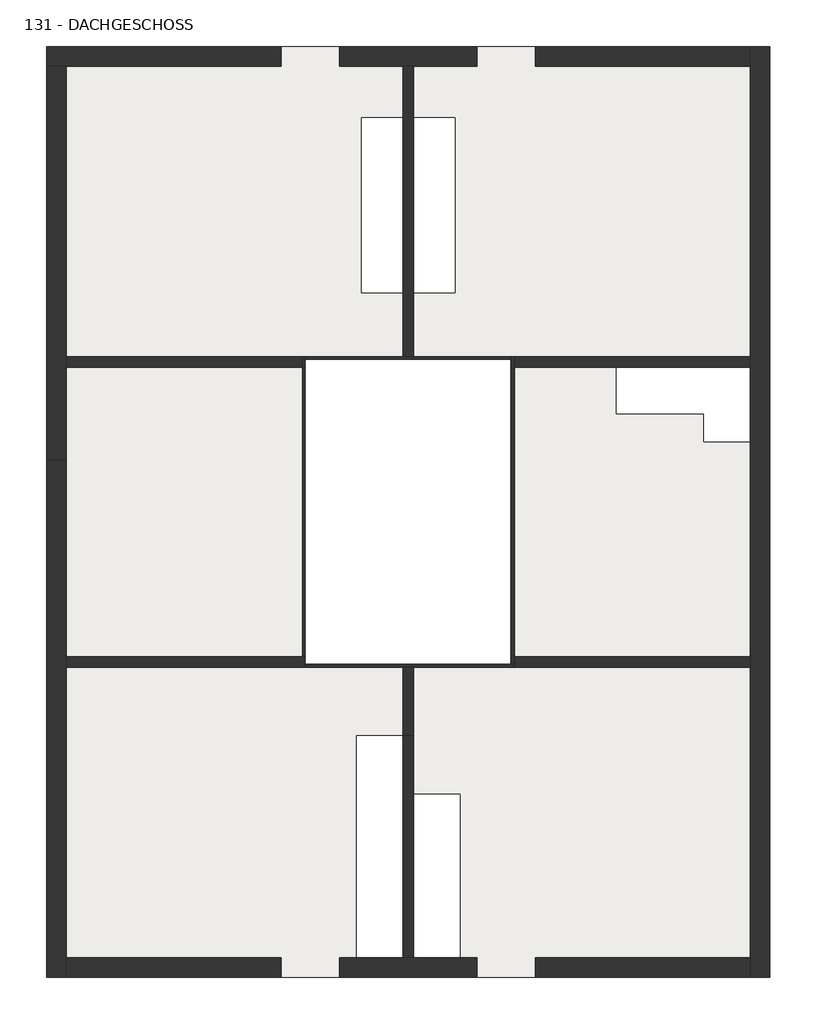
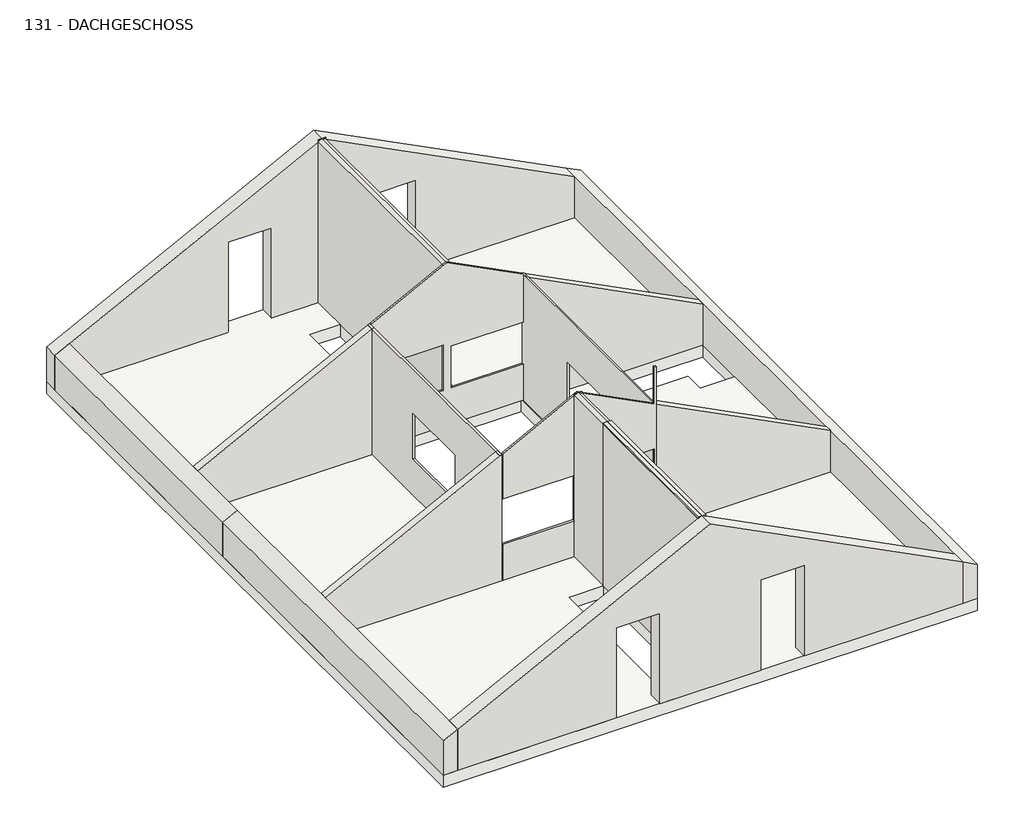
# One storey: 16 walls, 1 slab.
"""IFC4 building model written with IfcOpenShell, lengths in millimetres."""

import ifcopenshell
import ifcopenshell.guid

model = None  # the IFC model being written
_history = None  # IfcOwnerHistory: only IFC2X3 demands one
_inside = {}  # id of a spatial element -> (the spatial element, [elements in it])
_under = {}  # id of a project, library or spatial element -> (it, [spatial elements below it])
_declared = {}  # id of a project -> (the project, [libraries it declares])
_typed = {}  # id of a type object -> (the type object, [elements of that type])
_made_of = {}  # id of a material, layer set ... -> (it, [elements and type objects made of it])


def new_model(schema):
    """Start an empty IFC model of exactly this schema.

    Asked for "IFC4X3", IfcOpenShell would pick the latest addendum, in which some entities
    have other attributes; the version numbers below select the first issue.
    IFC2X3 requires an IfcOwnerHistory on every rooted entity: one is made here for all.
    """
    global model, _history
    if schema == "IFC4X3":
        model = ifcopenshell.file(schema_version=(4, 3, 0, 0))
    else:
        model = ifcopenshell.file(schema=schema)
    _inside.clear()
    _under.clear()
    _declared.clear()
    _typed.clear()
    _made_of.clear()
    _history = None
    if model.schema == "IFC2X3":
        org = make("IfcOrganization", Name="unknown")
        user = make(
            "IfcPersonAndOrganization",
            ThePerson=make("IfcPerson", FamilyName="unknown"),
            TheOrganization=org,
        )
        app = make(
            "IfcApplication",
            ApplicationDeveloper=org,
            Version="unknown",
            ApplicationFullName="unknown",
            ApplicationIdentifier="unknown",
        )
        _history = make(
            "IfcOwnerHistory",
            OwningUser=user,
            OwningApplication=app,
            ChangeAction="ADDED",
            CreationDate=0,
        )
    return model


def make(cls, **values):
    """One entity of the class cls with the attributes given. An attribute that is None is left unset."""
    return model.create_entity(
        cls, **{name: value for name, value in values.items() if value is not None}
    )


def rooted(cls, **values):
    """An entity with a GlobalId (a new one), such as an element, a storey or a relation."""
    return make(cls, GlobalId=ifcopenshell.guid.new(), OwnerHistory=_history, **values)


def si_unit(unit_type, name, prefix=None):
    """IfcSIUnit, for example si_unit("LENGTHUNIT", "METRE", prefix="MILLI")."""
    return make("IfcSIUnit", UnitType=unit_type, Prefix=prefix, Name=name)


def assignment(units):
    """IfcUnitAssignment: the units of a project."""
    return None if units is None else make("IfcUnitAssignment", Units=units)


def point(xyz):
    """IfcCartesianPoint."""
    return None if xyz is None else make("IfcCartesianPoint", Coordinates=xyz)


def direction(xyz):
    """IfcDirection."""
    return None if xyz is None else make("IfcDirection", DirectionRatios=xyz)


def frame(location, z_axis=None, x_axis=None):
    """IfcAxis2Placement3D, a coordinate frame: its origin and axes. An axis left out is left unset."""
    return make(
        "IfcAxis2Placement3D",
        Location=point(location),
        Axis=direction(z_axis),
        RefDirection=direction(x_axis),
    )


def origin():
    """The frame at (0, 0, 0) with its axes left unset."""
    return frame((0.0, 0.0, 0.0))


def place(relative_to, where):
    """IfcLocalPlacement: puts the frame where relative to a parent placement (None: the world)."""
    return make(
        "IfcLocalPlacement", PlacementRelTo=relative_to, RelativePlacement=where
    )


def context(
    kind, dimensions, precision=None, world=None, true_north=None, identifier=None
):
    """IfcGeometricRepresentationContext, for example the 3D "Model" context."""
    return make(
        "IfcGeometricRepresentationContext",
        ContextIdentifier=identifier,
        ContextType=kind,
        CoordinateSpaceDimension=dimensions,
        Precision=precision,
        WorldCoordinateSystem=world,
        TrueNorth=true_north,
    )


def project(units=None, contexts=None):
    """IfcProject with its units and contexts."""
    return rooted(
        "IfcProject",
        Name="project",
        RepresentationContexts=contexts,
        UnitsInContext=assignment(units),
    )


def spatial(cls, under=None, at=None, **own):
    """A site, building, storey or space (cls), placed at a placement, below another one or the project."""
    s = rooted(cls, ObjectPlacement=at, **own)
    if under is not None:
        _under.setdefault(under.id(), (under, []))[1].append(s)
    return s


def polyline(points):
    """IfcPolyline through the points."""
    return make("IfcPolyline", Points=[point(p) for p in points])


def outline(outer, holes=None, kind="AREA"):
    """IfcArbitraryClosedProfileDef: a profile drawn as a closed curve; with holes, ...WithVoids."""
    if holes is None:
        return make("IfcArbitraryClosedProfileDef", ProfileType=kind, OuterCurve=outer)
    return make(
        "IfcArbitraryProfileDefWithVoids",
        ProfileType=kind,
        OuterCurve=outer,
        InnerCurves=holes,
    )


def extrude(swept, where, along, depth):
    """IfcExtrudedAreaSolid: the profile swept, set in the frame where, extruded along a direction by depth."""
    return make(
        "IfcExtrudedAreaSolid",
        SweptArea=swept,
        Position=where,
        ExtrudedDirection=direction(along),
        Depth=depth,
    )


def faces_of(points, faces, orient=None, outer=None):
    """IfcFace entities. A face is a list of loops; a loop is a list of indices into points, from 0.

    orient and outer hold one flag for each loop. By default every Orientation is true, the
    first loop of a face is its IfcFaceOuterBound and the others are IfcFaceBound.
    """
    made = []
    for i, loops in enumerate(faces):
        bounds = []
        for j, loop in enumerate(loops):
            is_outer = j == 0 if outer is None else outer[i][j]
            bounds.append(
                make(
                    "IfcFaceOuterBound" if is_outer else "IfcFaceBound",
                    Bound=make("IfcPolyLoop", Polygon=[points[k] for k in loop]),
                    Orientation=True if orient is None else orient[i][j],
                )
            )
        made.append(make("IfcFace", Bounds=bounds))
    return made


def faceted_brep(points, faces, orient=None, outer=None, voids=None):
    """IfcFacetedBrep: a solid bounded by flat faces; with voids (closed shells), ...WithVoids."""
    shared = [point(p) for p in points]
    hull = make("IfcClosedShell", CfsFaces=faces_of(shared, faces, orient, outer))
    if voids is None:
        return make("IfcFacetedBrep", Outer=hull)
    return make(
        "IfcFacetedBrepWithVoids",
        Outer=hull,
        Voids=[
            make(cls, CfsFaces=faces_of(shared, fs, o, b)) for cls, fs, o, b in voids
        ],
    )


def shape(context_of_items, identifier, shape_type, items):
    """IfcShapeRepresentation: the items that make up one representation, for example the "Body"."""
    return make(
        "IfcShapeRepresentation",
        ContextOfItems=context_of_items,
        RepresentationIdentifier=identifier,
        RepresentationType=shape_type,
        Items=items,
    )


def source(mapping_origin, context_of_items, identifier, shape_type, items):
    """IfcRepresentationMap: a shape defined once, which mapped items show again and again."""
    return make(
        "IfcRepresentationMap",
        MappingOrigin=mapping_origin,
        MappedRepresentation=shape(context_of_items, identifier, shape_type, items),
    )


def transform(
    local_origin,
    x_axis=None,
    y_axis=None,
    z_axis=None,
    scale=None,
    scale2=None,
    scale3=None,
    uniform=True,
):
    """IfcCartesianTransformationOperator3D, or its non-uniform kind. x_axis, y_axis, z_axis: its Axis1, 2, 3."""
    if uniform:
        return make(
            "IfcCartesianTransformationOperator3D",
            Axis1=direction(x_axis),
            Axis2=direction(y_axis),
            LocalOrigin=point(local_origin),
            Scale=scale,
            Axis3=direction(z_axis),
        )
    return make(
        "IfcCartesianTransformationOperator3DnonUniform",
        Axis1=direction(x_axis),
        Axis2=direction(y_axis),
        LocalOrigin=point(local_origin),
        Scale=scale,
        Axis3=direction(z_axis),
        Scale2=scale2,
        Scale3=scale3,
    )


def mapped(mapping_source, mapping_target):
    """IfcMappedItem: shows the shape of a source again, moved by a transform."""
    return make(
        "IfcMappedItem", MappingSource=mapping_source, MappingTarget=mapping_target
    )


def made_of(thing, what):
    """Note that an element or type object is made of a material, layer set ...; save() writes the relation."""
    if what is not None:
        _made_of.setdefault(what.id(), (what, []))[1].append(thing)
    return thing


def element(
    cls,
    number,
    at=None,
    inside=None,
    cuts=None,
    type_object=None,
    material=None,
    context=None,
    identifier="Body",
    shape_type=None,
    held_by="IfcProductDefinitionShape",
    body=None,
    shapes=None,
    **own,
):
    """One element of the class cls, such as IfcWall. Its Tag is "e" and its number.

    at: its placement. inside: the storey or other place that contains it. cuts: it is an
    opening in that element (IfcRelVoidsElement). A single representation is given by context,
    identifier, shape_type and body (its items); several are given by shapes. held_by: the class
    of the entity that holds the representations. save() writes the other relations.
    """
    e = rooted(cls, Tag="e%d" % number, ObjectPlacement=at, **own)
    if body is not None:
        shapes = [shape(context, identifier, shape_type, body)]
    if shapes is not None:
        e.Representation = make(held_by, Representations=shapes)
    if inside is not None:
        _inside.setdefault(inside.id(), (inside, []))[1].append(e)
    if cuts is not None:
        rooted(
            "IfcRelVoidsElement", RelatingBuildingElement=cuts, RelatedOpeningElement=e
        )
    if type_object is not None:
        _typed.setdefault(type_object.id(), (type_object, []))[1].append(e)
    return made_of(e, material)


def aggregate(whole, parts):
    """IfcRelAggregates: a whole, such as a stair, and the parts it consists of."""
    return rooted("IfcRelAggregates", RelatingObject=whole, RelatedObjects=parts)


def save(model, path):
    """Write the relations noted so far, then the file.

    IfcRelAggregates (storeys below a building ...), IfcRelContainedInSpatialStructure (elements
    in a storey), IfcRelDefinesByType, IfcRelAssociatesMaterial and IfcRelDeclares: one each for
    every whole, place, type object, material and project.
    """
    for whole, parts in _under.values():
        aggregate(whole, parts)
    for where, things in _inside.values():
        rooted(
            "IfcRelContainedInSpatialStructure",
            RelatedElements=things,
            RelatingStructure=where,
        )
    for kind, things in _typed.values():
        rooted("IfcRelDefinesByType", RelatedObjects=things, RelatingType=kind)
    for what, things in _made_of.values():
        rooted("IfcRelAssociatesMaterial", RelatedObjects=things, RelatingMaterial=what)
    for by, libraries in _declared.values():
        rooted("IfcRelDeclares", RelatingContext=by, RelatedDefinitions=libraries)
    model.write(path)


def slab_52cff1b9(model_context):
    return source(origin(), model_context, "Body", "SweptSolid", [
        extrude(outline(polyline([(172797.7593015, 28481.9343946), (158797.7593015, 28481.9343946), (158797.7593015, 46484.7962965), (172797.7593015, 46484.7962965), (172797.7593015, 28481.9343946)]), holes=[polyline([(167772.7593015, 40484.7962965), (163772.7593015, 40484.7962965), (163772.7593015, 34484.7962965), (167772.7593015, 34484.7962965), (167772.7593015, 40484.7962965)]), polyline([(165697.7593015, 33159.7962965), (164797.7593015, 33159.7962965), (164797.7593015, 28861.9343946), (165697.7593015, 28861.9343946), (165697.7593015, 33159.7962965)]), polyline([(165897.7593015, 32021.9343946), (165897.7593015, 29779.7962965), (165897.7593015, 28861.9343946), (166797.7593015, 28861.9343946), (166797.7593015, 32021.9343946), (165897.7593015, 32021.9343946)]), polyline([(171517.7593015, 38844.7962965), (172417.7593015, 38844.7962965), (172417.7593015, 40284.7962965), (169822.7593015, 40284.7962965), (169822.7593015, 39384.7962965), (171517.7593015, 39384.7962965), (171517.7593015, 38844.7962965)]), polyline([(165897.7593015, 45104.7962965), (165897.7593015, 41724.7962965), (166697.7593015, 41724.7962965), (166697.7593015, 45104.7962965), (165897.7593015, 45104.7962965)]), polyline([(164897.7593015, 41724.7962965), (165697.7593015, 41724.7962965), (165697.7593015, 45104.7962965), (164897.7593015, 45104.7962965), (164897.7593015, 41724.7962965)])]), frame((0.0, 0.0, 5830.0), z_axis=(0.0, 0.0, 1.0), x_axis=(1.0, 0.0, 0.0)), (0.0, 0.0, 1.0), 330.0),
    ])


model = new_model("IFC4")

# Units and contexts
model_context = context("Model", 3, world=origin())
ifc_project = project(units=[si_unit("LENGTHUNIT", "METRE", prefix="MILLI")], contexts=[model_context])

# Site, building, storey
site = spatial("IfcSite", under=ifc_project)
building = spatial("IfcBuilding", under=site)
storey = spatial("IfcBuildingStorey", under=building, Name="131 - DACHGESCHOSS", Elevation=5650.0)

# Slab
placement = place(None, origin())
slab_shape = slab_52cff1b9(model_context)
element("IfcSlab", 1, ObjectType="Holzdecke 142136 : Holzdecke 142136", at=placement, inside=storey, context=model_context, shape_type="MappedRepresentation", body=[
    mapped(slab_shape, transform((0.0, 0.0, 0.0), x_axis=(1.0, 0.0, 0.0), y_axis=(0.0, 1.0, 0.0), z_axis=(0.0, 0.0, 1.0))),
])

# Walls
element("IfcWall", 2, ObjectType="Holzwand", at=placement, inside=storey, context=model_context, shape_type="SweptSolid", body=[
    extrude(outline(polyline([(6160.0, 167797.7593015), (6160.0, 172417.7593015), (7303.6196708, 172417.7593015), (9657.6272475, 167797.7593015), (6160.0, 167797.7593015)])), frame((0.0, 34484.7962965, 0.0), z_axis=(0.0, 1.0, 0.0), x_axis=(0.0, 0.0, 1.0)), (0.0, 0.0, 1.0), 200.0),
])
element("IfcWall", 3, ObjectType="Holzwand:1197", at=placement, inside=storey, context=model_context, shape_type="SweptSolid", body=[
    extrude(outline(polyline([(6160.0, 159177.7593015), (6160.0, 163797.7593015), (9657.6272475, 163797.7593015), (7303.6196708, 159177.7593015), (6160.0, 159177.7593015)])), frame((0.0, 34484.7962965, 0.0), z_axis=(0.0, 1.0, 0.0), x_axis=(0.0, 0.0, 1.0)), (0.0, 0.0, 1.0), 200.0),
])
element("IfcWall", 4, ObjectType="Holzwand:1195", at=placement, inside=storey, context=model_context, shape_type="SweptSolid", body=[
    extrude(outline(polyline([(6160.0, 167797.7593015), (6160.0, 172417.7593015), (7303.6196708, 172417.7593015), (9657.6272475, 167797.7593015), (6160.0, 167797.7593015)])), frame((0.0, 40284.7962965, 0.0), z_axis=(0.0, 1.0, 0.0), x_axis=(0.0, 0.0, 1.0)), (0.0, 0.0, 1.0), 200.0),
])
element("IfcWall", 5, ObjectType="Holzwand:1193", at=placement, inside=storey, context=model_context, shape_type="SweptSolid", body=[
    extrude(outline(polyline([(6160.0, 159177.7593015), (6160.0, 163797.7593015), (9657.6272475, 163797.7593015), (7303.6196708, 159177.7593015), (6160.0, 159177.7593015)])), frame((0.0, 40284.7962965, 0.0), z_axis=(0.0, 1.0, 0.0), x_axis=(0.0, 0.0, 1.0)), (0.0, 0.0, 1.0), 200.0),
])
element("IfcWall", 6, ObjectType=" ", at=placement, inside=storey, context=model_context, shape_type="Brep", body=[
    faceted_brep([(163797.7593015, 34484.7962965, 6160.0), (163797.7593015, 40484.7962965, 6160.0), (163797.7593015, 40484.7962965, 9657.6272475), (163797.7593015, 34484.7962965, 9657.6272475), (163797.7593015, 38434.7962965, 8420.0), (163797.7593015, 38434.7962965, 7160.0), (163797.7593015, 36534.7962965, 7160.0), (163797.7593015, 36534.7962965, 8420.0), (163747.7593015, 40484.7962965, 6160.0), (163747.7593015, 34484.7962965, 6160.0), (163747.7593015, 34484.7962965, 9632.150975), (163747.7593015, 40484.7962965, 9632.150975), (163747.7593015, 38434.7962965, 7160.0), (163747.7593015, 38434.7962965, 8420.0), (163747.7593015, 36534.7962965, 8420.0), (163747.7593015, 36534.7962965, 7160.0)], [[[0, 1, 2, 3], [4, 5, 6, 7]], [[8, 9, 10, 11], [12, 13, 14, 15]], [[1, 0, 9, 8]], [[2, 1, 8, 11]], [[0, 3, 10, 9]], [[3, 2, 11, 10]], [[4, 13, 12, 5]], [[13, 4, 7, 14]], [[14, 7, 6, 15]], [[5, 12, 15, 6]]]),
])
element("IfcWall", 7, ObjectType=" :1188", at=placement, inside=storey, context=model_context, shape_type="Brep", body=[
    faceted_brep([(167847.7593015, 34534.7962965, 6160.0), (163822.7593015, 34534.7962965, 6160.0), (163822.7593015, 34534.7962965, 7160.0), (165697.7593015, 34534.7962965, 7160.0), (165697.7593015, 34534.7962965, 8420.0), (163822.7593015, 34534.7962965, 8420.0), (163822.7593015, 34534.7962965, 9670.3653837), (165797.7593015, 34534.7962965, 10676.6781465), (167797.7593015, 34534.7962965, 9657.6272475), (167797.7593015, 34534.7962965, 10676.6781465), (167847.7593015, 34534.7962965, 10676.6781465), (165905.7229793, 34534.7962965, 8420.0), (165905.7229793, 34534.7962965, 7160.0), (167797.7593015, 34534.7962965, 7160.0), (167797.7593015, 34534.7962965, 8420.0), (163822.7593015, 34484.7962965, 6160.0), (167847.7593015, 34484.7962965, 6160.0), (167847.7593015, 34484.7962965, 10676.6781465), (167797.7593015, 34484.7962965, 10676.6781465), (167797.7593015, 34484.7962965, 9657.6272475), (165897.7593015, 34484.7962965, 10625.7256015), (165897.7593015, 34484.7962965, 10676.6781465), (165697.7593015, 34484.7962965, 10676.6781465), (165697.7593015, 34484.7962965, 10625.7256015), (163822.7593015, 34484.7962965, 9670.3653837), (163822.7593015, 34484.7962965, 8420.0), (165697.7593015, 34484.7962965, 8420.0), (165697.7593015, 34484.7962965, 7160.0), (163822.7593015, 34484.7962965, 7160.0), (165905.7229793, 34484.7962965, 7160.0), (165905.7229793, 34484.7962965, 8420.0), (167797.7593015, 34484.7962965, 8420.0), (167797.7593015, 34484.7962965, 7160.0), (165797.7593015, 34485.1993894, 10676.6781465)], [[[0, 1, 2, 3, 4, 5, 6, 7, 8, 9, 10], [11, 12, 13, 14]], [[15, 16, 17, 18, 19, 20, 21, 22, 23, 24, 25, 26, 27, 28], [29, 30, 31, 32]], [[1, 0, 16, 15]], [[1, 15, 28, 2]], [[24, 6, 5, 25]], [[17, 10, 9, 18]], [[22, 21, 33]], [[0, 10, 17, 16]], [[33, 20, 19, 8, 7]], [[20, 33, 21]], [[8, 19, 18, 9]], [[33, 7, 6, 24, 23]], [[33, 23, 22]], [[4, 26, 25, 5]], [[26, 4, 3, 27]], [[27, 3, 2, 28]], [[11, 30, 29, 12]], [[30, 11, 14, 31]], [[31, 14, 13, 32]], [[12, 29, 32, 13]]]),
])
element("IfcWall", 8, ObjectType=" :1186", at=placement, inside=storey, context=model_context, shape_type="Brep", body=[
    faceted_brep([(167797.7593015, 40484.7962965, 6160.0), (167797.7593015, 34484.7962965, 6160.0), (167797.7593015, 34484.7962965, 9657.6272475), (167797.7593015, 40484.7962965, 9657.6272475), (167797.7593015, 36534.7962965, 8420.0), (167797.7593015, 36534.7962965, 7160.0), (167797.7593015, 38434.7962965, 7160.0), (167797.7593015, 38434.7962965, 8420.0), (167847.7593015, 34484.7962965, 6160.0), (167847.7593015, 40484.7962965, 6160.0), (167847.7593015, 40484.7962965, 9632.150975), (167847.7593015, 34484.7962965, 9632.150975), (167847.7593015, 36534.7962965, 7160.0), (167847.7593015, 36534.7962965, 8420.0), (167847.7593015, 38434.7962965, 8420.0), (167847.7593015, 38434.7962965, 7160.0)], [[[0, 1, 2, 3], [4, 5, 6, 7]], [[8, 9, 10, 11], [12, 13, 14, 15]], [[1, 0, 9, 8]], [[2, 1, 8, 11]], [[0, 3, 10, 9]], [[3, 2, 11, 10]], [[12, 5, 4, 13]], [[13, 4, 7, 14]], [[14, 7, 6, 15]], [[5, 12, 15, 6]]]),
])
element("IfcWall", 9, ObjectType="Holzwand:1184", at=placement, inside=storey, context=model_context, shape_type="SweptSolid", body=[
    extrude(outline(polyline([(6160.0, 165697.7593015), (6160.0, 165897.7593015), (10625.7256015, 165897.7593015), (10676.6781465, 165797.7593015), (10625.7256015, 165697.7593015), (6160.0, 165697.7593015)])), frame((0.0, 28861.9343946, 0.0), z_axis=(0.0, 1.0, 0.0), x_axis=(0.0, 0.0, 1.0)), (0.0, 0.0, 1.0), 4297.8619019),
])
element("IfcWall", 10, ObjectType=" :1182", at=placement, inside=storey, context=model_context, shape_type="SweptSolid", body=[
    extrude(outline(polyline([(6160.0, 159177.7593015), (7303.6196708, 159177.7593015), (7110.0, 158797.7593015), (6160.0, 158797.7593015), (6160.0, 159177.7593015)])), frame((0.0, 28481.9343946, 0.0), z_axis=(0.0, 1.0, 0.0), x_axis=(0.0, 0.0, 1.0)), (0.0, 0.0, 1.0), 10002.8619019),
])
element("IfcWall", 11, ObjectType="Holzwand:1180", at=placement, inside=storey, context=model_context, shape_type="Brep", body=[
    faceted_brep([(165897.7593015, 40484.7962965, 6160.0), (165897.7593015, 46107.6581984, 6160.0), (165897.7593015, 46107.6581984, 10676.6781465), (165897.7593015, 46104.7962965, 10676.6781465), (165897.7593015, 46104.7962965, 10625.7256015), (165897.7593015, 40484.7962965, 10625.7256015), (165697.7593015, 46107.6581984, 6160.0), (165697.7593015, 40484.7962965, 6160.0), (165697.7593015, 40484.7962965, 10625.7256015), (165697.7593015, 46104.7962965, 10625.7256015), (165697.7593015, 46104.7962965, 10676.6781465), (165697.7593015, 46107.6581984, 10676.6781465), (165797.7593015, 46104.7962965, 10676.6781465), (165797.7593015, 40484.7962965, 10676.6781465)], [[[0, 1, 2, 3, 4, 5]], [[6, 7, 8, 9, 10, 11]], [[1, 0, 7, 6]], [[2, 1, 6, 11]], [[2, 11, 10, 12, 3]], [[7, 0, 5, 13, 8]], [[4, 12, 13, 5]], [[12, 4, 3]], [[9, 12, 10]], [[13, 12, 9, 8]]]),
])
element("IfcWall", 12, ObjectType="Holzwand:1178", at=placement, inside=storey, context=model_context, shape_type="Brep", body=[
    faceted_brep([(165897.7593015, 28862.3374874, 6160.0), (165897.7593015, 34485.1993894, 6160.0), (165897.7593015, 34485.1993894, 10625.7256015), (165897.7593015, 33159.7962965, 10625.7256015), (165897.7593015, 33159.7962965, 10676.6781465), (165897.7593015, 28862.3374874, 10676.6781465), (165697.7593015, 34485.1993894, 6160.0), (165697.7593015, 28862.3374874, 6160.0), (165697.7593015, 28862.3374874, 10676.6781465), (165697.7593015, 33159.7962965, 10676.6781465), (165697.7593015, 33159.7962965, 10625.7256015), (165697.7593015, 34485.1993894, 10625.7256015), (165797.7593015, 34485.1993894, 10676.6781465), (165797.7593015, 33159.7962965, 10676.6781465)], [[[0, 1, 2, 3, 4, 5]], [[6, 7, 8, 9, 10, 11]], [[1, 0, 7, 6]], [[1, 6, 11, 12, 2]], [[8, 5, 4, 13, 9]], [[0, 5, 8, 7]], [[13, 3, 2, 12]], [[3, 13, 4]], [[13, 10, 9]], [[13, 12, 11, 10]]]),
])
element("IfcWall", 13, ObjectType=" :1176", at=placement, inside=storey, context=model_context, shape_type="SweptSolid", body=[
    extrude(outline(polyline([(7303.6196708, 172417.7593015), (6160.0, 172417.7593015), (6160.0, 172797.7593015), (7110.0, 172797.7593015), (7303.6196708, 172417.7593015)])), frame((0.0, 28481.9343946, 0.0), z_axis=(0.0, 1.0, 0.0), x_axis=(0.0, 0.0, 1.0)), (0.0, 0.0, 1.0), 18002.8619019),
])
element("IfcWall", 14, ObjectType=" :1174", at=placement, inside=storey, context=model_context, shape_type="SweptSolid", body=[
    extrude(outline(polyline([(6160.0, 159177.7593015), (7303.6196708, 159177.7593015), (7110.0, 158797.7593015), (6160.0, 158797.7593015), (6160.0, 159177.7593015)])), frame((0.0, 38484.7962965, 0.0), z_axis=(0.0, 1.0, 0.0), x_axis=(0.0, 0.0, 1.0)), (0.0, 0.0, 1.0), 7620.0),
])
element("IfcWall", 15, ObjectType=" :1190", at=placement, inside=storey, context=model_context, shape_type="SweptSolid", body=[
    extrude(outline(polyline([(6160.0, 163797.7593015), (6160.0, 167797.7593015), (7160.0, 167797.7593015), (7160.0, 165897.7593015), (8320.0, 165897.7593015), (8320.0, 167797.7593015), (9657.6272475, 167797.7593015), (10676.6781465, 165797.7593015), (9657.6272475, 163797.7593015), (8420.0, 163797.7593015), (8420.0, 165697.7593015), (7160.0, 165697.7593015), (7160.0, 163797.7593015), (6160.0, 163797.7593015)])), frame((0.0, 40434.7962965, 0.0), z_axis=(0.0, 1.0, 0.0), x_axis=(0.0, 0.0, 1.0)), (0.0, 0.0, 1.0), 50.0),
])
element("IfcWall", 16, ObjectType=" :1201", at=placement, inside=storey, context=model_context, shape_type="SweptSolid", body=[
    extrude(outline(polyline([(7303.6196708, 159177.7593015), (6160.0, 159177.7593015), (6160.0, 163337.7593015), (8660.0, 163337.7593015), (8660.0, 164472.7593015), (6160.0, 164472.7593015), (6160.0, 167122.7593015), (8660.0, 167122.7593015), (8660.0, 168257.7593015), (6160.0, 168257.7593015), (6160.0, 172417.7593015), (7303.6196708, 172417.7593015), (10676.6781465, 165797.7593015), (7303.6196708, 159177.7593015)])), frame((0.0, 28481.9343946, 0.0), z_axis=(0.0, 1.0, 0.0), x_axis=(0.0, 0.0, 1.0)), (0.0, 0.0, 1.0), 380.0),
])
element("IfcWall", 17, ObjectType=" :1202", at=placement, inside=storey, context=model_context, shape_type="SweptSolid", body=[
    extrude(outline(polyline([(6160.0, 172417.7593015), (7303.6196708, 172417.7593015), (10676.6781465, 165797.7593015), (7110.0, 158797.7593015), (6160.0, 158797.7593015), (6160.0, 163337.7593015), (8660.0, 163337.7593015), (8660.0, 164472.7593015), (6160.0, 164472.7593015), (6160.0, 167122.7593015), (8660.0, 167122.7593015), (8660.0, 168257.7593015), (6160.0, 168257.7593015), (6160.0, 172417.7593015)])), frame((0.0, 46104.7962965, 0.0), z_axis=(0.0, 1.0, 0.0), x_axis=(0.0, 0.0, 1.0)), (0.0, 0.0, 1.0), 380.0),
])

save(model, "model.ifc")

# Revit data of these elements
# Type "Holzdecke 142136 : Holzdecke 142136"
#   Abrechnungsart = "m²"
#   Allright_Bauteil_ID = "0123De 0783954319"
#   Bezeichnung = "Holzdecke"
#   Codetext = "D-HOLZBALKEN1\\"
#   Gewerk = "Zimmer- und Holzbauarbeiten"
#   Material = "Holz"
#   Objektname = "Brettstapeldecke"
#   NameOverride = "Holzdecke"
#   Reference = "Holzdecke"
#   Status = "NEW"
#   PitchAngle = 0.00°
#   ThermalTransmittance = 0.0000 BTU/(h·ft²·°F)
#   2D Interaktion = yes
#   Combustible = no
#   Compartmentation = no
#   IsExternal = no
#   LoadBearing = yes
# Type "Holzwand"
#   ThermalTransmittance = 0.0000 BTU/(h·ft²·°F)
#   Combustible = no
#   Compartmentation = no
#   Layers, outside or top first: 0.200 m "holzschalung" (function 1)
# Type "Holzwand:1197"
#   ThermalTransmittance = 0.0000 BTU/(h·ft²·°F)
#   Combustible = no
#   Compartmentation = no
#   Layers, outside or top first: 0.200 m "holzschalung" (function 1)
# Type "Holzwand:1195"
#   ThermalTransmittance = 0.0000 BTU/(h·ft²·°F)
#   Combustible = no
#   Compartmentation = no
#   Layers, outside or top first: 0.200 m "holzschalung" (function 1)
# Type "Holzwand:1193"
#   ThermalTransmittance = 0.0000 BTU/(h·ft²·°F)
#   Combustible = no
#   Compartmentation = no
#   Layers, outside or top first: 0.200 m "holzschalung" (function 1)
# Type " "
#   Layers, outside or top first: 0.050 m "holzschalung" (function 1)
# Type " :1188"
#   Layers, outside or top first: 0.050 m "holzschalung" (function 1)
# Type " :1186"
#   Layers, outside or top first: 0.050 m "holzschalung" (function 1)
# Type "Holzwand:1184"
#   ThermalTransmittance = 0.0000 BTU/(h·ft²·°F)
#   Combustible = no
#   Compartmentation = no
#   Layers, outside or top first: 0.200 m "holzschalung" (function 1)
# Type " :1182"
#   Layers, outside or top first: 0.380 m "holzschalung" (function 1)
# Type "Holzwand:1180"
#   ThermalTransmittance = 0.0000 BTU/(h·ft²·°F)
#   Combustible = no
#   Compartmentation = no
#   Layers, outside or top first: 0.200 m "holzschalung" (function 1)
# Type "Holzwand:1178"
#   ThermalTransmittance = 0.0000 BTU/(h·ft²·°F)
#   Combustible = no
#   Compartmentation = no
#   Layers, outside or top first: 0.200 m "holzschalung" (function 1)
# Type " :1176"
#   Layers, outside or top first: 0.380 m "holzschalung" (function 1)
# Type " :1174"
#   Layers, outside or top first: 0.380 m "holzschalung" (function 1)
# Type " :1190"
#   Layers, outside or top first: 0.050 m "holzschalung" (function 1)
# Type " :1201"
#   Layers, outside or top first: 0.380 m "holzschalung" (function 1)
# Type " :1202"
#   Layers, outside or top first: 0.380 m "holzschalung" (function 1)
# Element 1 (IfcSlab, "Holzdecke 142136 : Holzdecke 142136")
#   IFC Predefined Type = "FLOOR"
#   Export to IFC As = "ifcslab"
#   IfcGUID = "2UFX_hum15ZQP8rfQ2hTBa"
#   Phase Created = New Construction
#   Materials on its faces: "holzschalung"
# Element 2 (IfcWall, "Holzwand")
#   Export to IFC As = "ifcwall"
#   IfcGUID = "2irPo0fN95hwd6nGWO8xKX"
#   NameOverride = "Holzwand"
#   Abrechnungsart = "St"
#   Allright_Bauteil_ID = "0131HWa0658953274"
#   Bezeichnung = "Holzwand"
#   Layer #1:Object Layer Attributes #1:Abrechnungsart = "m²"
#   Layer #1:Object Layer Attributes #1:Allright_Bauteil_ID = "0131Wa 0658953275"
#   Layer #1:Object Layer Attributes #1:Bezeichnung = "Holzwand"
#   Layer #1:Object Layer Attributes #1:Codetext = "HO-WI-HSW\\"
#   Layer #1:Object Layer Attributes #1:Gewerk = "Zimmer- und Holzbauarbeiten"
#   Layer #1:Object Layer Attributes #1:Material = "Holz"
#   Layer #1:Object Layer Attributes #1:Objektname = "Wand"
#   Layer #1:Object Layer Attributes #1:Reference = "Holzwand"
#   Layer #1:Object Layer Attributes #1:Status = "Neubau"
#   MEP Wandtyp = "HO-WA-HSW\\"
#   Objektname = "Gesamtwand"
#   Reference = "Holzwand"
#   Status = "NEW"
#   built-in parameter 1001111 = 0.510 m
#   Top Offset = 0.000 m
#   Base Offset = 0.510 m
#   Unconnected Height = 3.497627 m
#   wall height = 3.497627 m
#   Layer #1:Object Layer Attributes #1:U-Wert = 0
#   Layer #1:Object Layer Attributes #1:2D Interaktion = yes
#   Layer #1:Object Layer Attributes #1:Außenbauteil = no
#   Layer #1:Object Layer Attributes #1:Brandabschnittsdefinierendes Bauteil = no
#   Layer #1:Object Layer Attributes #1:Brennbares Material = no
#   Layer #1:Object Layer Attributes #1:Raumhohe Wand = yes
#   Layer #1:Object Layer Attributes #1:Tragendes Bauteil = yes
#   ExtendToStructure = yes
#   IsExternal = no
#   LoadBearing = yes
#   Phase Created = New Construction
#   Base Constraint = 131 - DACHGESCHOSS
#   Materials on its faces: "holzschalung"
# Element 3 (IfcWall, "Holzwand:1197")
#   Export to IFC As = "ifcwall"
#   IfcGUID = "0btdfUgAf1BODjBN4XyqI6"
#   NameOverride = "Holzwand"
#   Abrechnungsart = "St"
#   Allright_Bauteil_ID = "0131HWa0658955859"
#   Bezeichnung = "Holzwand"
#   Layer #1:Object Layer Attributes #1:Abrechnungsart = "m²"
#   Layer #1:Object Layer Attributes #1:Allright_Bauteil_ID = "0131Wa 0658955860"
#   Layer #1:Object Layer Attributes #1:Bezeichnung = "Holzwand"
#   Layer #1:Object Layer Attributes #1:Codetext = "HO-WI-HSW\\"
#   Layer #1:Object Layer Attributes #1:Gewerk = "Zimmer- und Holzbauarbeiten"
#   Layer #1:Object Layer Attributes #1:Material = "Holz"
#   Layer #1:Object Layer Attributes #1:Objektname = "Wand"
#   Layer #1:Object Layer Attributes #1:Reference = "Holzwand"
#   Layer #1:Object Layer Attributes #1:Status = "Neubau"
#   MEP Wandtyp = "HO-WA-HSW\\"
#   Objektname = "Gesamtwand"
#   Reference = "Holzwand"
#   Status = "NEW"
#   built-in parameter 1001111 = 0.510 m
#   Top Offset = 0.000 m
#   Base Offset = 0.510 m
#   Unconnected Height = 3.497627 m
#   wall height = 3.497627 m
#   Layer #1:Object Layer Attributes #1:U-Wert = 0
#   Layer #1:Object Layer Attributes #1:2D Interaktion = yes
#   Layer #1:Object Layer Attributes #1:Außenbauteil = no
#   Layer #1:Object Layer Attributes #1:Brandabschnittsdefinierendes Bauteil = no
#   Layer #1:Object Layer Attributes #1:Brennbares Material = no
#   Layer #1:Object Layer Attributes #1:Raumhohe Wand = yes
#   Layer #1:Object Layer Attributes #1:Tragendes Bauteil = yes
#   ExtendToStructure = yes
#   IsExternal = no
#   LoadBearing = yes
#   Phase Created = New Construction
#   Base Constraint = 131 - DACHGESCHOSS
#   Materials on its faces: "holzschalung"
# Element 4 (IfcWall, "Holzwand:1195")
#   Export to IFC As = "ifcwall"
#   IfcGUID = "2RQ2xt8jL3z9U7Ow04WNfJ"
#   NameOverride = "Holzwand"
#   Abrechnungsart = "St"
#   Allright_Bauteil_ID = "0131HWa0658953259"
#   Bezeichnung = "Holzwand"
#   Layer #1:Object Layer Attributes #1:Abrechnungsart = "m²"
#   Layer #1:Object Layer Attributes #1:Allright_Bauteil_ID = "0131Wa 0658953260"
#   Layer #1:Object Layer Attributes #1:Bezeichnung = "Holzwand"
#   Layer #1:Object Layer Attributes #1:Codetext = "HO-WI-HSW\\"
#   Layer #1:Object Layer Attributes #1:Gewerk = "Zimmer- und Holzbauarbeiten"
#   Layer #1:Object Layer Attributes #1:Material = "Holz"
#   Layer #1:Object Layer Attributes #1:Objektname = "Wand"
#   Layer #1:Object Layer Attributes #1:Reference = "Holzwand"
#   Layer #1:Object Layer Attributes #1:Status = "Neubau"
#   MEP Wandtyp = "HO-WA-HSW\\"
#   Objektname = "Gesamtwand"
#   Reference = "Holzwand"
#   Status = "NEW"
#   built-in parameter 1001111 = 0.510 m
#   Top Offset = 0.000 m
#   Base Offset = 0.510 m
#   Unconnected Height = 3.497627 m
#   wall height = 3.497627 m
#   Layer #1:Object Layer Attributes #1:U-Wert = 0
#   Layer #1:Object Layer Attributes #1:2D Interaktion = yes
#   Layer #1:Object Layer Attributes #1:Außenbauteil = no
#   Layer #1:Object Layer Attributes #1:Brandabschnittsdefinierendes Bauteil = no
#   Layer #1:Object Layer Attributes #1:Brennbares Material = no
#   Layer #1:Object Layer Attributes #1:Raumhohe Wand = yes
#   Layer #1:Object Layer Attributes #1:Tragendes Bauteil = yes
#   ExtendToStructure = yes
#   IsExternal = no
#   LoadBearing = yes
#   Phase Created = New Construction
#   Base Constraint = 131 - DACHGESCHOSS
#   Materials on its faces: "holzschalung"
# Element 5 (IfcWall, "Holzwand:1193")
#   Export to IFC As = "ifcwall"
#   IfcGUID = "1XDlXo4IT97OvdyoFppHWZ"
#   NameOverride = "Holzwand"
#   Abrechnungsart = "St"
#   Allright_Bauteil_ID = "0131HWa0658952486"
#   Bezeichnung = "Holzwand"
#   Layer #1:Object Layer Attributes #1:Abrechnungsart = "m²"
#   Layer #1:Object Layer Attributes #1:Allright_Bauteil_ID = "0131Wa 0658952490"
#   Layer #1:Object Layer Attributes #1:Bezeichnung = "Holzwand"
#   Layer #1:Object Layer Attributes #1:Codetext = "HO-WI-HSW\\"
#   Layer #1:Object Layer Attributes #1:Gewerk = "Zimmer- und Holzbauarbeiten"
#   Layer #1:Object Layer Attributes #1:Material = "Holz"
#   Layer #1:Object Layer Attributes #1:Objektname = "Wand"
#   Layer #1:Object Layer Attributes #1:Reference = "Holzwand"
#   Layer #1:Object Layer Attributes #1:Status = "Neubau"
#   MEP Wandtyp = "HO-WA-HSW\\"
#   Objektname = "Gesamtwand"
#   Reference = "Holzwand"
#   Status = "NEW"
#   built-in parameter 1001111 = 0.510 m
#   Top Offset = 0.000 m
#   Base Offset = 0.510 m
#   Unconnected Height = 3.497627 m
#   wall height = 3.497627 m
#   Layer #1:Object Layer Attributes #1:U-Wert = 0
#   Layer #1:Object Layer Attributes #1:2D Interaktion = yes
#   Layer #1:Object Layer Attributes #1:Außenbauteil = no
#   Layer #1:Object Layer Attributes #1:Brandabschnittsdefinierendes Bauteil = no
#   Layer #1:Object Layer Attributes #1:Brennbares Material = no
#   Layer #1:Object Layer Attributes #1:Raumhohe Wand = yes
#   Layer #1:Object Layer Attributes #1:Tragendes Bauteil = yes
#   ExtendToStructure = yes
#   IsExternal = no
#   LoadBearing = yes
#   Phase Created = New Construction
#   Base Constraint = 131 - DACHGESCHOSS
#   Materials on its faces: "holzschalung"
# Element 6 (IfcWall, " ")
#   Export to IFC As = "ifcwall"
#   IfcGUID = "21FF_DgHzF28s1dzPXnAcl"
#   NameOverride = " "
#   Abrechnungsart = "m³"
#   Allright_Bauteil_ID = "0131HWa0658952409"
#   Layer #1:Object Layer Attributes #1:Abrechnungsart = "m²"
#   Layer #1:Object Layer Attributes #1:Allright_Bauteil_ID = "0131Wa 0658952493"
#   Layer #1:Object Layer Attributes #1:Gewerk = "Zimmer- und Holzbauarbeiten"
#   Layer #1:Object Layer Attributes #1:Material = "k.Ausw."
#   Layer #1:Object Layer Attributes #1:Objektname = "Wand"
#   Layer #1:Object Layer Attributes #1:Status = "Neubau"
#   MEP Wandtyp = "HO-WA-HSW\\"
#   Objektname = "Gesamtwand"
#   built-in parameter 1001111 = 0.510 m
#   Top Offset = 0.000 m
#   Base Offset = 0.510 m
#   Unconnected Height = 3.497627 m
#   wall height = 3.497627 m
#   Layer #1:Object Layer Attributes #1:2D Interaktion = yes
#   Phase Created = New Construction
#   Base Constraint = 131 - DACHGESCHOSS
#   Materials on its faces: "holzschalung"
# Element 7 (IfcWall, " :1188")
#   Export to IFC As = "ifcwall"
#   IfcGUID = "1sDERupobB$8G6O8zmS_FC"
#   NameOverride = " "
#   Abrechnungsart = "m³"
#   Allright_Bauteil_ID = "0131HWa0658952407"
#   Layer #1:Object Layer Attributes #1:Abrechnungsart = "m²"
#   Layer #1:Object Layer Attributes #1:Allright_Bauteil_ID = "0131Wa 0658952497"
#   Layer #1:Object Layer Attributes #1:Gewerk = "Zimmer- und Holzbauarbeiten"
#   Layer #1:Object Layer Attributes #1:Material = "k.Ausw."
#   Layer #1:Object Layer Attributes #1:Objektname = "Wand"
#   Layer #1:Object Layer Attributes #1:Status = "Neubau"
#   MEP Wandtyp = "HO-WA-HSW\\"
#   Objektname = "Gesamtwand"
#   built-in parameter 1001111 = 0.510 m
#   Top Offset = 0.000 m
#   Base Offset = 0.510 m
#   Unconnected Height = 4.516678 m
#   wall height = 4.516678 m
#   Layer #1:Object Layer Attributes #1:2D Interaktion = yes
#   Phase Created = New Construction
#   Base Constraint = 131 - DACHGESCHOSS
#   Materials on its faces: "holzschalung"
# Element 8 (IfcWall, " :1186")
#   Export to IFC As = "ifcwall"
#   IfcGUID = "2vPa_8WInC1fLjRjt9C8qD"
#   NameOverride = " "
#   Abrechnungsart = "m³"
#   Allright_Bauteil_ID = "0131HWa0658952411"
#   Layer #1:Object Layer Attributes #1:Abrechnungsart = "m²"
#   Layer #1:Object Layer Attributes #1:Allright_Bauteil_ID = "0131Wa 0658952482"
#   Layer #1:Object Layer Attributes #1:Gewerk = "Zimmer- und Holzbauarbeiten"
#   Layer #1:Object Layer Attributes #1:Material = "k.Ausw."
#   Layer #1:Object Layer Attributes #1:Objektname = "Wand"
#   Layer #1:Object Layer Attributes #1:Status = "Neubau"
#   MEP Wandtyp = "HO-WA-HSW\\"
#   Objektname = "Gesamtwand"
#   built-in parameter 1001111 = 0.510 m
#   Top Offset = 0.000 m
#   Base Offset = 0.510 m
#   Unconnected Height = 3.497627 m
#   wall height = 3.497627 m
#   Layer #1:Object Layer Attributes #1:2D Interaktion = yes
#   Phase Created = New Construction
#   Base Constraint = 131 - DACHGESCHOSS
#   Materials on its faces: "holzschalung"
# Element 9 (IfcWall, "Holzwand:1184")
#   Export to IFC As = "ifcwall"
#   IfcGUID = "3sGwvbH0X0wRT5LbxtOghV"
#   NameOverride = "Holzwand"
#   Abrechnungsart = "St"
#   Allright_Bauteil_ID = "0131HWa0658956028"
#   Bezeichnung = "Holzwand"
#   Layer #1:Object Layer Attributes #1:Abrechnungsart = "m²"
#   Layer #1:Object Layer Attributes #1:Allright_Bauteil_ID = "0131Wa 0658956031"
#   Layer #1:Object Layer Attributes #1:Bezeichnung = "Holzwand"
#   Layer #1:Object Layer Attributes #1:Codetext = "HO-WI-HSW\\"
#   Layer #1:Object Layer Attributes #1:Gewerk = "Zimmer- und Holzbauarbeiten"
#   Layer #1:Object Layer Attributes #1:Material = "Holz"
#   Layer #1:Object Layer Attributes #1:Objektname = "Wand"
#   Layer #1:Object Layer Attributes #1:Reference = "Holzwand"
#   Layer #1:Object Layer Attributes #1:Status = "Neubau"
#   MEP Wandtyp = "HO-WA-HSW\\"
#   Objektname = "Gesamtwand"
#   Reference = "Holzwand"
#   Status = "NEW"
#   built-in parameter 1001111 = 0.510 m
#   Top Offset = 0.000 m
#   Base Offset = 0.510 m
#   Unconnected Height = 4.516678 m
#   wall height = 4.516678 m
#   Layer #1:Object Layer Attributes #1:U-Wert = 0
#   Layer #1:Object Layer Attributes #1:2D Interaktion = yes
#   Layer #1:Object Layer Attributes #1:Außenbauteil = no
#   Layer #1:Object Layer Attributes #1:Brandabschnittsdefinierendes Bauteil = no
#   Layer #1:Object Layer Attributes #1:Brennbares Material = no
#   Layer #1:Object Layer Attributes #1:Raumhohe Wand = yes
#   Layer #1:Object Layer Attributes #1:Tragendes Bauteil = yes
#   ExtendToStructure = yes
#   IsExternal = no
#   LoadBearing = yes
#   Phase Created = New Construction
#   Base Constraint = 131 - DACHGESCHOSS
#   Materials on its faces: "holzschalung"
# Element 10 (IfcWall, " :1182")
#   Export to IFC As = "ifcwall"
#   IfcGUID = "2d5_L$AAv1WBYQkgHyHFrb"
#   NameOverride = " "
#   Abrechnungsart = "m³"
#   Allright_Bauteil_ID = "0131HWa0658952452"
#   Layer #1:Object Layer Attributes #1:Abrechnungsart = "m²"
#   Layer #1:Object Layer Attributes #1:Allright_Bauteil_ID = "0131Wa 0658952457"
#   Layer #1:Object Layer Attributes #1:Gewerk = "Zimmer- und Holzbauarbeiten"
#   Layer #1:Object Layer Attributes #1:Material = "k.Ausw."
#   Layer #1:Object Layer Attributes #1:Objektname = "Wand"
#   Layer #1:Object Layer Attributes #1:Status = "Neubau"
#   MEP Wandtyp = "HO-WA-HSW\\"
#   Objektname = "Gesamtwand"
#   built-in parameter 1001111 = 0.510 m
#   Top Offset = 0.000 m
#   Base Offset = 0.510 m
#   Unconnected Height = 1.14362 m
#   wall height = 1.14362 m
#   Layer #1:Object Layer Attributes #1:2D Interaktion = yes
#   Phase Created = New Construction
#   Base Constraint = 131 - DACHGESCHOSS
#   Materials on its faces: "holzschalung"
# Element 11 (IfcWall, "Holzwand:1180")
#   Export to IFC As = "ifcwall"
#   IfcGUID = "1F6NxEW8b7hgcJafh_mgpg"
#   NameOverride = "Holzwand"
#   Abrechnungsart = "St"
#   Allright_Bauteil_ID = "0131HWa0658952466"
#   Bezeichnung = "Holzwand"
#   Layer #1:Object Layer Attributes #1:Abrechnungsart = "m²"
#   Layer #1:Object Layer Attributes #1:Allright_Bauteil_ID = "0131Wa 0658952469"
#   Layer #1:Object Layer Attributes #1:Bezeichnung = "Holzwand"
#   Layer #1:Object Layer Attributes #1:Codetext = "HO-WI-HSW\\"
#   Layer #1:Object Layer Attributes #1:Gewerk = "Zimmer- und Holzbauarbeiten"
#   Layer #1:Object Layer Attributes #1:Material = "Holz"
#   Layer #1:Object Layer Attributes #1:Objektname = "Wand"
#   Layer #1:Object Layer Attributes #1:Reference = "Holzwand"
#   Layer #1:Object Layer Attributes #1:Status = "Neubau"
#   MEP Wandtyp = "HO-WA-HSW\\"
#   Objektname = "Gesamtwand"
#   Reference = "Holzwand"
#   Status = "NEW"
#   built-in parameter 1001111 = 0.510 m
#   Top Offset = 0.000 m
#   Base Offset = 0.510 m
#   Unconnected Height = 4.516678 m
#   wall height = 4.516678 m
#   Layer #1:Object Layer Attributes #1:U-Wert = 0
#   Layer #1:Object Layer Attributes #1:2D Interaktion = yes
#   Layer #1:Object Layer Attributes #1:Außenbauteil = no
#   Layer #1:Object Layer Attributes #1:Brandabschnittsdefinierendes Bauteil = no
#   Layer #1:Object Layer Attributes #1:Brennbares Material = no
#   Layer #1:Object Layer Attributes #1:Raumhohe Wand = yes
#   Layer #1:Object Layer Attributes #1:Tragendes Bauteil = yes
#   ExtendToStructure = yes
#   IsExternal = no
#   LoadBearing = yes
#   Phase Created = New Construction
#   Base Constraint = 131 - DACHGESCHOSS
#   Materials on its faces: "holzschalung"
# Element 12 (IfcWall, "Holzwand:1178")
#   Export to IFC As = "ifcwall"
#   IfcGUID = "00NikNq3z8kAwJn0xK23rS"
#   NameOverride = "Holzwand"
#   Abrechnungsart = "St"
#   Allright_Bauteil_ID = "0131HWa0658952460"
#   Bezeichnung = "Holzwand"
#   Layer #1:Object Layer Attributes #1:Abrechnungsart = "m²"
#   Layer #1:Object Layer Attributes #1:Allright_Bauteil_ID = "0131Wa 0658952463"
#   Layer #1:Object Layer Attributes #1:Bezeichnung = "Holzwand"
#   Layer #1:Object Layer Attributes #1:Codetext = "HO-WI-HSW\\"
#   Layer #1:Object Layer Attributes #1:Gewerk = "Zimmer- und Holzbauarbeiten"
#   Layer #1:Object Layer Attributes #1:Material = "Holz"
#   Layer #1:Object Layer Attributes #1:Objektname = "Wand"
#   Layer #1:Object Layer Attributes #1:Reference = "Holzwand"
#   Layer #1:Object Layer Attributes #1:Status = "Neubau"
#   MEP Wandtyp = "HO-WA-HSW\\"
#   Objektname = "Gesamtwand"
#   Reference = "Holzwand"
#   Status = "NEW"
#   built-in parameter 1001111 = 0.510 m
#   Top Offset = 0.000 m
#   Base Offset = 0.510 m
#   Unconnected Height = 4.516678 m
#   wall height = 4.516678 m
#   Layer #1:Object Layer Attributes #1:U-Wert = 0
#   Layer #1:Object Layer Attributes #1:2D Interaktion = yes
#   Layer #1:Object Layer Attributes #1:Außenbauteil = no
#   Layer #1:Object Layer Attributes #1:Brandabschnittsdefinierendes Bauteil = no
#   Layer #1:Object Layer Attributes #1:Brennbares Material = no
#   Layer #1:Object Layer Attributes #1:Raumhohe Wand = yes
#   Layer #1:Object Layer Attributes #1:Tragendes Bauteil = yes
#   ExtendToStructure = yes
#   IsExternal = no
#   LoadBearing = yes
#   Phase Created = New Construction
#   Base Constraint = 131 - DACHGESCHOSS
#   Materials on its faces: "holzschalung"
# Element 13 (IfcWall, " :1176")
#   Export to IFC As = "ifcwall"
#   IfcGUID = "0ZVIYFQNr0sP3ZyLP7_6Tg"
#   NameOverride = " "
#   Abrechnungsart = "m³"
#   Allright_Bauteil_ID = "0131HWa0658952403"
#   Layer #1:Object Layer Attributes #1:Abrechnungsart = "m²"
#   Layer #1:Object Layer Attributes #1:Allright_Bauteil_ID = "0131Wa 0658952478"
#   Layer #1:Object Layer Attributes #1:Gewerk = "Zimmer- und Holzbauarbeiten"
#   Layer #1:Object Layer Attributes #1:Material = "k.Ausw."
#   Layer #1:Object Layer Attributes #1:Objektname = "Wand"
#   Layer #1:Object Layer Attributes #1:Status = "Neubau"
#   MEP Wandtyp = "HO-WA-HSW\\"
#   Objektname = "Gesamtwand"
#   built-in parameter 1001111 = 0.510 m
#   Top Offset = 0.000 m
#   Base Offset = 0.510 m
#   Unconnected Height = 1.14362 m
#   wall height = 1.14362 m
#   Layer #1:Object Layer Attributes #1:2D Interaktion = yes
#   Phase Created = New Construction
#   Base Constraint = 131 - DACHGESCHOSS
#   Materials on its faces: "holzschalung"
# Element 14 (IfcWall, " :1174")
#   Export to IFC As = "ifcwall"
#   IfcGUID = "3U9_YM0ybA1AScTQjjWjui"
#   NameOverride = " "
#   Abrechnungsart = "m³"
#   Allright_Bauteil_ID = "0131HWa0658952400"
#   Layer #1:Object Layer Attributes #1:Abrechnungsart = "m²"
#   Layer #1:Object Layer Attributes #1:Allright_Bauteil_ID = "0131Wa 0658952488"
#   Layer #1:Object Layer Attributes #1:Gewerk = "Zimmer- und Holzbauarbeiten"
#   Layer #1:Object Layer Attributes #1:Material = "k.Ausw."
#   Layer #1:Object Layer Attributes #1:Objektname = "Wand"
#   Layer #1:Object Layer Attributes #1:Status = "Neubau"
#   MEP Wandtyp = "HO-WA-HSW\\"
#   Objektname = "Gesamtwand"
#   built-in parameter 1001111 = 0.510 m
#   Top Offset = 0.000 m
#   Base Offset = 0.510 m
#   Unconnected Height = 1.14362 m
#   wall height = 1.14362 m
#   Layer #1:Object Layer Attributes #1:2D Interaktion = yes
#   Phase Created = New Construction
#   Base Constraint = 131 - DACHGESCHOSS
#   Materials on its faces: "holzschalung"
# Element 15 (IfcWall, " :1190")
#   Export to IFC As = "ifcwall"
#   IfcGUID = "3Ip91QNbHFI9IYnpBcAhv9"
#   NameOverride = " "
#   Abrechnungsart = "m³"
#   Allright_Bauteil_ID = "0131HWa0658952413"
#   Layer #1:Object Layer Attributes #1:Abrechnungsart = "m²"
#   Layer #1:Object Layer Attributes #1:Allright_Bauteil_ID = "0131Wa 0658952495"
#   Layer #1:Object Layer Attributes #1:Gewerk = "Zimmer- und Holzbauarbeiten"
#   Layer #1:Object Layer Attributes #1:Material = "k.Ausw."
#   Layer #1:Object Layer Attributes #1:Objektname = "Wand"
#   Layer #1:Object Layer Attributes #1:Status = "Neubau"
#   MEP Wandtyp = "HO-WA-HSW\\"
#   Objektname = "Gesamtwand"
#   built-in parameter 1001111 = 0.510 m
#   Top Offset = 0.000 m
#   Base Offset = 0.510 m
#   Unconnected Height = 4.516678 m
#   wall height = 4.516678 m
#   Layer #1:Object Layer Attributes #1:2D Interaktion = yes
#   Phase Created = New Construction
#   Base Constraint = 131 - DACHGESCHOSS
#   Materials on its faces: "holzschalung"
# Element 16 (IfcWall, " :1201")
#   Export to IFC As = "ifcwall"
#   IfcGUID = "2WTZnHm_rA_vN8rU_4QeBZ"
#   NameOverride = " "
#   Abrechnungsart = "m³"
#   Allright_Bauteil_ID = "0131HWa0658952415"
#   Layer #1:Object Layer Attributes #1:Abrechnungsart = "m²"
#   Layer #1:Object Layer Attributes #1:Allright_Bauteil_ID = "0131Wa 0658952451"
#   Layer #1:Object Layer Attributes #1:Gewerk = "Zimmer- und Holzbauarbeiten"
#   Layer #1:Object Layer Attributes #1:Material = "k.Ausw."
#   Layer #1:Object Layer Attributes #1:Objektname = "Wand"
#   Layer #1:Object Layer Attributes #1:Status = "Neubau"
#   MEP Wandtyp = "HO-WA-HSW\\"
#   Objektname = "Gesamtwand"
#   built-in parameter 1001111 = 0.510 m
#   Top Offset = 0.000 m
#   Base Offset = 0.510 m
#   Unconnected Height = 4.516678 m
#   wall height = 4.516678 m
#   Layer #1:Object Layer Attributes #1:2D Interaktion = yes
#   Phase Created = New Construction
#   Base Constraint = 131 - DACHGESCHOSS
#   Materials on its faces: "holzschalung"
# Element 17 (IfcWall, " :1202")
#   Export to IFC As = "ifcwall"
#   IfcGUID = "00rhRKdfT8yut5ruNEaTcS"
#   NameOverride = " "
#   Abrechnungsart = "m³"
#   Allright_Bauteil_ID = "0131HWa0659067833"
#   Layer #1:Object Layer Attributes #1:Abrechnungsart = "m²"
#   Layer #1:Object Layer Attributes #1:Allright_Bauteil_ID = "0131Wa 0659067848"
#   Layer #1:Object Layer Attributes #1:Gewerk = "Zimmer- und Holzbauarbeiten"
#   Layer #1:Object Layer Attributes #1:Material = "k.Ausw."
#   Layer #1:Object Layer Attributes #1:Objektname = "Wand"
#   Layer #1:Object Layer Attributes #1:Status = "Neubau"
#   MEP Wandtyp = "HO-WA-HSW\\"
#   Objektname = "Gesamtwand"
#   built-in parameter 1001111 = 0.510 m
#   Top Offset = 0.000 m
#   Base Offset = 0.510 m
#   Unconnected Height = 4.516678 m
#   wall height = 4.516678 m
#   Layer #1:Object Layer Attributes #1:2D Interaktion = yes
#   Phase Created = New Construction
#   Base Constraint = 131 - DACHGESCHOSS
#   Materials on its faces: "holzschalung"
# Materials
#   "holzschalung": class "Unassigned", colour RGB 128 128 128, transparency 0
# Room at (167757.171, 31673.18) mm, phase "New Construction", upper offset 9.610411 m, lower offset 0.000 m
#   Export to IFC As = "ifcspace"
#   IfcGUID = "28AMI5zSb64OR5RJn7fYQN"
#   Comments = ""
#   Number = "37"
#   Name = "Galerie 3"
#   Abrechnungsart = "m²"
#   Allright_Bauteil_ID = "0131Rau0659044724"
#   Objektname = "Raum"
#   Status = "Neubau"
#   Flächenart_DIN277 = "N"
#   Flächenart_Wohnfläche = "WO"
#   Nutzungsart_Din277 = "NUF"
#   Ortscode_Geschoßbezeichnung = "OG"
#   Raumumschließung = "R"
#   Faktor_DIN277 = 1
#   Faktor_Wohnfläche_Raum = 1
#   BauNVO_Anrechnung_auf_GF = 0
#   BauNVO_Anrechnung_auf_GR = 0
#   Raum unter Treppe (Wohnfl erst ab 2m) = 0
# Room at (169265.802, 36444.087) mm, phase "New Construction", upper offset 7.996768 m, lower offset 0.000 m
#   Export to IFC As = "ifcspace"
#   IfcGUID = "01Tq8ih5D6yPFZ$HlcW1vc"
#   Comments = ""
#   Number = "38"
#   Name = "Galerie 4"
#   Abrechnungsart = "m²"
#   Allright_Bauteil_ID = "0131Rau0658956932"
#   Objektname = "Raum"
#   Status = "Neubau"
#   Flächenart_DIN277 = "N"
#   Flächenart_Wohnfläche = "WO"
#   Nutzungsart_Din277 = "NUF"
#   Ortscode_Geschoßbezeichnung = "OG"
#   Raumumschließung = "R"
#   Faktor_DIN277 = 1
#   Faktor_Wohnfläche_Raum = 1
#   BauNVO_Anrechnung_auf_GF = 0
#   BauNVO_Anrechnung_auf_GR = 0
#   Raum unter Treppe (Wohnfl erst ab 2m) = 0
# Room at (167757.171, 43294.796) mm, phase "New Construction", upper offset 9.608458 m, lower offset 0.000 m
#   Export to IFC As = "ifcspace"
#   IfcGUID = "3tbBfsSpX5Ch0OjDEnzAkE"
#   Comments = ""
#   Number = "39"
#   Name = "Galerie 5"
#   Abrechnungsart = "m²"
#   Allright_Bauteil_ID = "0131Rau0658957290"
#   Objektname = "Raum"
#   Status = "Neubau"
#   Flächenart_DIN277 = "N"
#   Flächenart_Wohnfläche = "WO"
#   Nutzungsart_Din277 = "NUF"
#   Ortscode_Geschoßbezeichnung = "OG"
#   Raumumschließung = "R"
#   Faktor_DIN277 = 1
#   Faktor_Wohnfläche_Raum = 1
#   BauNVO_Anrechnung_auf_GF = 0
#   BauNVO_Anrechnung_auf_GR = 0
#   Raum unter Treppe (Wohnfl erst ab 2m) = 0
# Room at (161638.476, 43442.554) mm, phase "New Construction", upper offset 9.608458 m, lower offset 0.000 m
#   Export to IFC As = "ifcspace"
#   IfcGUID = "1DRA1FAkPCIxabdWTo2FhX"
#   Comments = ""
#   Number = "40"
#   Name = "Galerie 6"
#   Abrechnungsart = "m²"
#   Allright_Bauteil_ID = "0131Rau0658957330"
#   Objektname = "Raum"
#   Status = "Neubau"
#   Flächenart_DIN277 = "N"
#   Flächenart_Wohnfläche = "WO"
#   Nutzungsart_Din277 = "NUF"
#   Ortscode_Geschoßbezeichnung = "OG"
#   Raumumschließung = "R"
#   Faktor_DIN277 = 1
#   Faktor_Wohnfläche_Raum = 1
#   BauNVO_Anrechnung_auf_GF = 0
#   BauNVO_Anrechnung_auf_GR = 0
#   Raum unter Treppe (Wohnfl erst ab 2m) = 0
# Room at (161638.476, 30472.232) mm, phase "New Construction", upper offset 9.610187 m, lower offset 0.000 m
#   Export to IFC As = "ifcspace"
#   IfcGUID = "0HHBQQ6NrEHhnLM8NG$h5T"
#   Comments = ""
#   Number = "41"
#   Name = "Galerie 2"
#   Abrechnungsart = "m²"
#   Allright_Bauteil_ID = "0131Rau0659044691"
#   Objektname = "Raum"
#   Status = "Neubau"
#   Flächenart_DIN277 = "N"
#   Flächenart_Wohnfläche = "WO"
#   Nutzungsart_Din277 = "NUF"
#   Ortscode_Geschoßbezeichnung = "OG"
#   Raumumschließung = "R"
#   Faktor_DIN277 = 1
#   Faktor_Wohnfläche_Raum = 1
#   BauNVO_Anrechnung_auf_GF = 0
#   BauNVO_Anrechnung_auf_GR = 0
#   Raum unter Treppe (Wohnfl erst ab 2m) = 0
# Room at (162329.717, 36444.087) mm, phase "New Construction", upper offset 7.996768 m, lower offset 0.000 m
#   Export to IFC As = "ifcspace"
#   IfcGUID = "3PlIdw6HzF0gMclH3ThgTL"
#   Comments = ""
#   Number = "42"
#   Name = "Galerie 7"
#   Abrechnungsart = "m²"
#   Allright_Bauteil_ID = "0131Rau0658957043"
#   Objektname = "Raum"
#   Status = "Neubau"
#   Flächenart_DIN277 = "N"
#   Flächenart_Wohnfläche = "WO"
#   Nutzungsart_Din277 = "NUF"
#   Ortscode_Geschoßbezeichnung = "OG"
#   Raumumschließung = "R"
#   Faktor_DIN277 = 1
#   Faktor_Wohnfläche_Raum = 1
#   BauNVO_Anrechnung_auf_GF = 0
#   BauNVO_Anrechnung_auf_GR = 0
#   Raum unter Treppe (Wohnfl erst ab 2m) = 0
